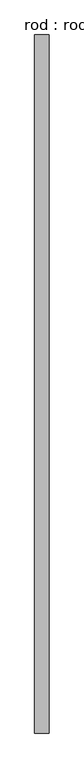
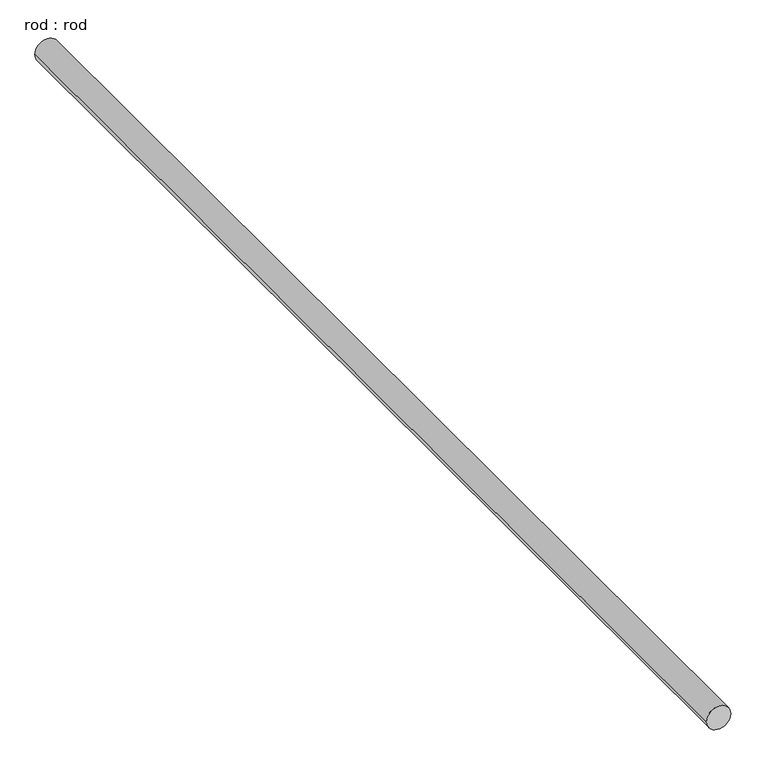
"""IFC4 building model written with IfcOpenShell, lengths in millimetres: proxy geometry, rod : rod."""

from ifc_helpers import new_model, si_unit, point, frame, frame_2d, origin, place, context, project, spatial, circle_curve, trimmed, segment, composite_curve, outline, extrude, source, transform, mapped, element, save


def rod_rod_179da68a(model_context):
    return source(origin(), model_context, "Body", "SweptSolid", [
        extrude(outline(composite_curve([segment(trimmed(circle_curve(frame_2d((0.0108462, 0.0)), 200.0), [point((0.0108462, 200.0))], [point((0.0108462, -200.0))], False, "CARTESIAN"), True, "CONTINUOUS"), segment(trimmed(circle_curve(frame_2d((0.0108462, 0.0)), 200.0), [point((0.0108462, -200.0))], [point((0.0108462, 200.0))], False, "CARTESIAN"), True, "CONTINUOUS")], self_intersect=False)), frame((0.0, -5482.0102845, 0.0), z_axis=(0.0, 1.0, 0.0), x_axis=(0.0, 0.0, 1.0)), (0.0, 0.0, 1.0), 19149.4777997),
    ])


if __name__ == "__main__":
    model = new_model("IFC4")
    model_context = context("Model", 3, world=origin())
    ifc_project = project(units=[si_unit("LENGTHUNIT", "METRE", prefix="MILLI")], contexts=[model_context])
    site = spatial("IfcSite", under=ifc_project)
    building = spatial("IfcBuilding", under=site)
    placement = place(None, origin())
    rod_rod_shape = rod_rod_179da68a(model_context)
    element("IfcBuildingElementProxy", 1, Name="rod : rod", ObjectType="rod : rod", at=placement, inside=building, context=model_context, shape_type="MappedRepresentation", body=[
        mapped(rod_rod_shape, transform((0.0, 0.0, 0.0), x_axis=(1.0, 0.0, 0.0), y_axis=(0.0, 1.0, 0.0), z_axis=(0.0, 0.0, 1.0))),
    ])
    save(model, "model.ifc")

# Revit data of these elements
# Type "rod : rod"
#   Default Elevation = 0
